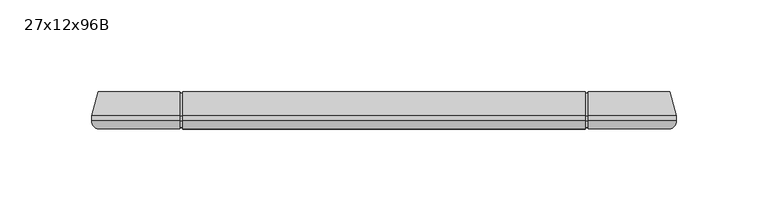
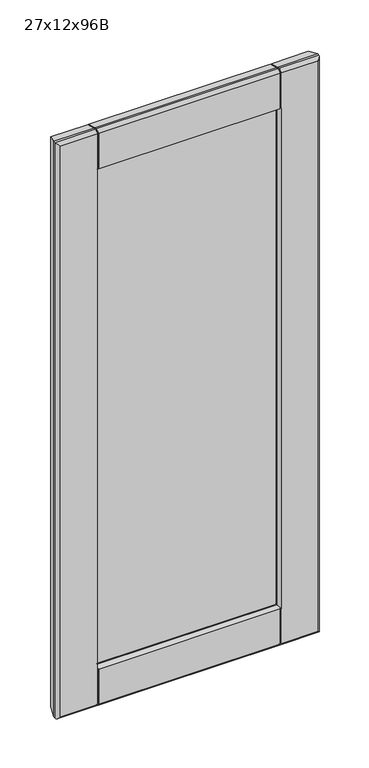
"""IFC4 building model written with IfcOpenShell, lengths in millimetres: furniture geometry, Cabinet-Tall-Merillat-Utility_Double-Marlin : 27x12x96B."""

from ifc_helpers import new_model, si_unit, frame, origin, place, context, project, spatial, polyline, circle_curve, ellipse_curve, outline, extrude, source, transform, mapped, element, save
from ifc_brep_helpers import plane_surface, cylinder_surface, advanced_brep


def furniture_27x12x96b_cd454a86(model_context):
    return source(origin(), model_context, "Body", "SolidModel", [
        advanced_brep(
        [(-326.6853408, -320.6496, 1676.4), (-323.5888483, -325.12, 1679.4964925), (-323.5888483, -325.12, 2409.9035075), (-326.6853408, -320.6496, 2413.0), (-326.6853408, -317.881, 2413.0), (-326.6853408, -317.881, 1676.4), (-323.1801408, -304.8, 2409.4948), (-323.1801408, -304.8, 1679.9052), (-278.4841781, -304.8, 1724.6011628), (-278.4841781, -304.8, 2364.7988372), (-278.1140464, -305.59375, 2364.4287055), (-276.0328873, -310.05681, 2362.3475465), (-276.0328873, -310.05681, 1727.0524535), (-278.1140464, -305.59375, 1724.9712945), (-277.4326568, -312.2969093, 2363.747316), (-277.4326568, -312.2969093, 1725.652684), (-291.7603408, -312.547, 2378.075), (-291.7603408, -312.547, 1711.325), (-291.7603408, -317.373, 2378.075), (-291.7603408, -317.373, 1711.325), (-277.4326568, -317.6230907, 2363.747316), (-277.4326568, -317.6230907, 1725.652684), (-276.0328873, -319.86319, 2362.3475465), (-276.0328873, -319.86319, 1727.0524535), (-278.1140464, -324.32625, 2364.4287055), (-278.4813106, -325.1138508, 2364.7959698), (-278.4841781, -325.12, 1724.6011628), (-278.1140464, -324.32625, 1724.9712945), (-278.4813106, -325.12, 2409.9035075), (-278.4813106, -320.6496, 2413.0), (-10.6943333, -325.12, 2409.9035075), (-7.5978408, -320.6496, 2413.0), (-55.7620595, -320.6496, 2413.0), (-55.7620595, -325.12, 2409.9035075), (-276.8938106, -320.6496, 2413.0), (-276.8938106, -325.12, 2409.9035075), (-57.3495595, -325.12, 2409.9035075), (-57.3495595, -320.6496, 2413.0), (-278.4813106, -317.881, 2413.0), (-7.5978408, -317.881, 2413.0), (-55.7620595, -317.881, 2413.0), (-276.8938106, -317.881, 2413.0), (-57.3495595, -317.881, 2413.0), (-278.4813106, -304.8, 2409.4948), (-11.1030408, -304.8, 2409.4948), (-55.7620595, -304.8, 2409.4948), (-276.8938106, -304.8, 2409.4948), (-57.3495595, -304.8, 2409.4948), (-58.2502943, -310.05681, 2362.3475465), (-276.8938106, -305.59375, 2364.4287055), (-276.8938106, -304.8, 2364.7988372), (-57.3495595, -304.8, 2364.7988372), (-57.3495595, -305.59375, 2364.4287055), (-56.1691353, -305.59375, 2364.4287055), (-56.8505249, -312.2969093, 2363.747316), (-42.5228408, -312.547, 2378.075), (-42.5228408, -317.373, 2378.075), (-56.8505249, -317.6230907, 2363.747316), (-58.2502943, -319.86319, 2362.3475465), (-56.1691353, -324.32625, 2364.4287055), (-57.3495595, -324.32625, 2364.4287055), (-57.3495595, -325.12, 2364.7988372), (-276.8938106, -325.12, 2364.7988372), (-276.8938106, -324.32625, 2364.4287055), (-10.6943333, -325.12, 1679.4964925), (-7.5978408, -320.6496, 1676.4), (-7.5978408, -317.881, 1676.4), (-11.1030408, -304.8, 1679.9052), (-55.7990036, -304.8, 2364.7988372), (-55.7990036, -304.8, 1724.6011628), (-56.1691353, -305.59375, 1724.9712945), (-58.2502943, -310.05681, 1727.0524535), (-56.8505249, -312.2969093, 1725.652684), (-42.5228408, -312.547, 1711.325), (-42.5228408, -317.373, 1711.325), (-56.8505249, -317.6230907, 1725.652684), (-58.2502943, -319.86319, 1727.0524535), (-56.1691353, -324.32625, 1724.9712945), (-55.7990036, -325.12, 1724.6011628), (-55.7990036, -325.12, 2364.7988372), (-55.7620595, -325.12, 1679.4964925), (-55.7620595, -320.6496, 1676.4), (-278.4813106, -320.6496, 1676.4), (-278.4813106, -325.12, 1679.4964925), (-57.3495595, -320.6496, 1676.4), (-57.3495595, -325.12, 1679.4964925), (-276.8938106, -325.12, 1679.4964925), (-276.8938106, -320.6496, 1676.4), (-55.7620595, -317.881, 1676.4), (-278.4813106, -317.881, 1676.4), (-57.3495595, -317.881, 1676.4), (-276.8938106, -317.881, 1676.4), (-55.7620595, -304.8, 1679.9052), (-278.4813106, -304.8, 1679.9052), (-57.3495595, -304.8, 1679.9052), (-276.8938106, -304.8, 1679.9052), (-57.3495595, -304.8, 1724.6011628), (-276.8938106, -304.8, 1724.6011628), (-57.3495595, -305.59375, 1724.9712945), (-276.8938106, -305.59375, 1724.9712945), (-276.8938106, -324.32625, 1724.9712945), (-276.8938106, -325.12, 1724.6011628), (-57.3495595, -325.12, 1724.6011628), (-57.3495595, -324.32625, 1724.9712945), (-57.3495595, -305.59375, 1680.5142588), (-57.3495595, -317.9855037, 1677.19375), (-57.3495595, -320.6496, 1677.19375), (-57.3495595, -324.32625, 1679.6473948), (-55.7620595, -324.32625, 1724.9712945), (-55.7620595, -324.32625, 1679.6473948), (-55.7620595, -320.6496, 1677.19375), (-55.7620595, -317.9855037, 1677.19375), (-55.7620595, -305.59375, 1680.5142588), (-55.7620595, -305.59375, 1724.9712945), (-278.4813106, -305.59375, 1724.9712945), (-278.4813106, -305.59375, 1680.5142588), (-278.4813106, -317.9855037, 1677.19375), (-278.4813106, -320.6496, 1677.19375), (-278.4813106, -324.32625, 1679.6473948), (-278.4813106, -324.32625, 1724.9712945), (-276.8938106, -324.32625, 1679.6473948), (-276.8938106, -320.6496, 1677.19375), (-276.8938106, -317.9855037, 1677.19375), (-276.8938106, -305.59375, 1680.5142588), (-278.4813106, -324.32625, 2364.4287055), (-278.4813106, -324.32625, 2409.7526052), (-278.4813106, -320.6496, 2412.20625), (-278.4813106, -317.9855037, 2412.20625), (-278.4813106, -305.59375, 2408.8857412), (-278.4813106, -305.59375, 2364.4287055), (-276.8938106, -305.59375, 2408.8857412), (-276.8938106, -317.9855037, 2412.20625), (-276.8938106, -320.6496, 2412.20625), (-276.8938106, -324.32625, 2409.7526052), (-57.3495595, -324.32625, 2409.7526052), (-57.3495595, -320.6496, 2412.20625), (-57.3495595, -317.9855037, 2412.20625), (-57.3495595, -305.59375, 2408.8857412), (-55.7620595, -324.32625, 2364.4287055), (-55.7620595, -305.59375, 2364.4287055), (-55.7620595, -305.59375, 2408.8857412), (-55.7620595, -317.9855037, 2412.20625), (-55.7620595, -320.6496, 2412.20625), (-55.7620595, -324.32625, 2409.7526052)],
        [
            (0, 1, ellipse_curve(frame((-321.9101408, -320.6496, 1681.1752), z_axis=(-0.7071067811865505, 0.0, 0.7071067811865446), x_axis=(-0.7071067811865445, 0.0, -0.7071067811865505)), 6.7531526, 4.7752)),
            (1, 2),
            (2, 3, ellipse_curve(frame((-321.9101408, -320.6496, 2408.2248), z_axis=(-0.7071067811865446, 0.0, -0.7071067811865505), x_axis=(0.7071067811865505, 0.0, -0.7071067811865445)), 6.7531526, 4.7752)),
            (3, 0),
            (3, 4),
            (4, 5),
            (5, 0),
            (4, 6),
            (6, 7),
            (7, 5),
            (8, 9),
            (9, 10),
            (10, 11),
            (11, 12),
            (12, 13),
            (13, 8),
            (11, 14, ellipse_curve(frame((-277.4601408, -310.7223492, 2363.7748), z_axis=(-0.7071067811865446, 0.0, -0.7071067811865505), x_axis=(0.7071067811865505, 0.0, -0.7071067811865445)), 2.2271035, 1.5748)),
            (14, 15),
            (15, 12, ellipse_curve(frame((-277.4601408, -310.7223492, 1725.6252), z_axis=(-0.7071067811865505, 0.0, 0.7071067811865446), x_axis=(-0.7071067811865445, 0.0, -0.7071067811865505)), 2.2271035, 1.5748)),
            (14, 16),
            (16, 17),
            (17, 15),
            (16, 18),
            (18, 19),
            (19, 17),
            (18, 20),
            (20, 21),
            (21, 19),
            (20, 22, ellipse_curve(frame((-277.4601408, -319.1976508, 2363.7748), z_axis=(-0.7071067811865446, 0.0, -0.7071067811865505), x_axis=(0.7071067811865505, 0.0, -0.7071067811865445)), 2.2271035, 1.5748)),
            (22, 23),
            (23, 21, ellipse_curve(frame((-277.4601408, -319.1976508, 1725.6252), z_axis=(-0.7071067811865505, 0.0, 0.7071067811865446), x_axis=(-0.7071067811865445, 0.0, -0.7071067811865505)), 2.2271035, 1.5748)),
            (22, 24),
            (24, 25),
            (25, 26),
            (26, 27),
            (27, 23),
            (2, 28),
            (28, 29, circle_curve(frame((-278.4813106, -320.6496, 2408.2248), z_axis=(-1.0, 0.0, 0.0), x_axis=(0.0, 1.0, 0.0)), 4.7752)),
            (29, 3),
            (30, 31, ellipse_curve(frame((-12.3730408, -320.6496, 2408.2248), z_axis=(-0.7071067811865505, 0.0, 0.7071067811865446), x_axis=(-0.7071067811865445, 0.0, -0.7071067811865505)), 6.7531526, 4.7752)),
            (31, 32),
            (32, 33, circle_curve(frame((-55.7620595, -320.6496, 2408.2248), z_axis=(1.0, 0.0, 0.0), x_axis=(0.0, 1.0, 0.0)), 4.7752)),
            (33, 30),
            (34, 35, circle_curve(frame((-276.8938106, -320.6496, 2408.2248), z_axis=(1.0, 0.0, 0.0), x_axis=(0.0, 1.0, 0.0)), 4.7752)),
            (35, 36),
            (36, 37, circle_curve(frame((-57.3495595, -320.6496, 2408.2248), z_axis=(-1.0, 0.0, 0.0), x_axis=(0.0, 1.0, 0.0)), 4.7752)),
            (37, 34),
            (29, 38),
            (38, 4),
            (31, 39),
            (39, 40),
            (40, 32),
            (41, 34),
            (37, 42),
            (42, 41),
            (38, 43),
            (43, 6),
            (39, 44),
            (44, 45),
            (45, 40),
            (46, 41),
            (42, 47),
            (47, 46),
            (48, 11),
            (10, 49),
            (49, 50),
            (50, 51),
            (51, 52),
            (52, 53),
            (53, 48),
            (48, 54, ellipse_curve(frame((-56.8230408, -310.7223492, 2363.7748), z_axis=(-0.7071067811865505, 0.0, 0.7071067811865446), x_axis=(-0.7071067811865445, 0.0, -0.7071067811865505)), 2.2271035, 1.5748)),
            (54, 14),
            (54, 55),
            (55, 16),
            (55, 56),
            (56, 18),
            (56, 57),
            (57, 20),
            (57, 58, ellipse_curve(frame((-56.8230408, -319.1976508, 2363.7748), z_axis=(-0.7071067811865505, 0.0, 0.7071067811865446), x_axis=(-0.7071067811865445, 0.0, -0.7071067811865505)), 2.2271035, 1.5748)),
            (58, 22),
            (58, 59),
            (59, 60),
            (60, 61),
            (61, 62),
            (62, 63),
            (63, 24),
            (30, 64),
            (64, 65, ellipse_curve(frame((-12.3730408, -320.6496, 1681.1752), z_axis=(0.7071067811865446, 0.0, 0.7071067811865505), x_axis=(-0.7071067811865505, 0.0, 0.7071067811865445)), 6.7531526, 4.7752)),
            (65, 31),
            (65, 66),
            (66, 39),
            (66, 67),
            (67, 44),
            (68, 69),
            (69, 70),
            (70, 71),
            (71, 48),
            (53, 68),
            (71, 72, ellipse_curve(frame((-56.8230408, -310.7223492, 1725.6252), z_axis=(0.7071067811865446, 0.0, 0.7071067811865505), x_axis=(-0.7071067811865505, 0.0, 0.7071067811865445)), 2.2271035, 1.5748)),
            (72, 54),
            (72, 73),
            (73, 55),
            (73, 74),
            (74, 56),
            (74, 75),
            (75, 57),
            (75, 76, ellipse_curve(frame((-56.8230408, -319.1976508, 1725.6252), z_axis=(0.7071067811865446, 0.0, 0.7071067811865505), x_axis=(-0.7071067811865505, 0.0, 0.7071067811865445)), 2.2271035, 1.5748)),
            (76, 58),
            (76, 77),
            (77, 78),
            (78, 79),
            (79, 59),
            (64, 80),
            (80, 81, circle_curve(frame((-55.7620595, -320.6496, 1681.1752), z_axis=(1.0, 0.0, 0.0), x_axis=(0.0, 1.0, 0.0)), 4.7752)),
            (81, 65),
            (0, 82),
            (82, 83, circle_curve(frame((-278.4813106, -320.6496, 1681.1752), z_axis=(-1.0, 0.0, 0.0), x_axis=(0.0, 1.0, 0.0)), 4.7752)),
            (83, 1),
            (84, 85, circle_curve(frame((-57.3495595, -320.6496, 1681.1752), z_axis=(-1.0, 0.0, 0.0), x_axis=(0.0, 1.0, 0.0)), 4.7752)),
            (85, 86),
            (86, 87, circle_curve(frame((-276.8938106, -320.6496, 1681.1752), z_axis=(1.0, 0.0, 0.0), x_axis=(0.0, 1.0, 0.0)), 4.7752)),
            (87, 84),
            (81, 88),
            (88, 66),
            (5, 89),
            (89, 82),
            (90, 84),
            (87, 91),
            (91, 90),
            (88, 92),
            (92, 67),
            (7, 93),
            (93, 89),
            (94, 90),
            (91, 95),
            (95, 94),
            (43, 9),
            (8, 93),
            (92, 69),
            (68, 45),
            (96, 94),
            (95, 97),
            (97, 96),
            (50, 46),
            (47, 51),
            (12, 71),
            (70, 98),
            (98, 96),
            (97, 99),
            (99, 13),
            (15, 72),
            (17, 73),
            (19, 74),
            (21, 75),
            (23, 76),
            (27, 100),
            (100, 101),
            (101, 102),
            (102, 103),
            (103, 77),
            (83, 26),
            (25, 28),
            (33, 79),
            (78, 80),
            (85, 102),
            (101, 86),
            (35, 62),
            (61, 36),
            (98, 104),
            (104, 105),
            (105, 106),
            (106, 107, circle_curve(frame((-57.3495595, -320.6496, 1681.1752), z_axis=(-1.0, 0.0, 0.0), x_axis=(0.0, 0.0, -1.0)), 3.98145)),
            (107, 103),
            (78, 108),
            (108, 109),
            (109, 110, circle_curve(frame((-55.7620595, -320.6496, 1681.1752), z_axis=(1.0, 0.0, 0.0), x_axis=(0.0, 0.0, -1.0)), 3.98145)),
            (110, 111),
            (111, 112),
            (112, 113),
            (113, 69),
            (77, 108),
            (107, 109),
            (106, 110),
            (105, 111),
            (104, 112),
            (70, 113),
            (8, 114),
            (114, 115),
            (115, 116),
            (116, 117),
            (117, 118, circle_curve(frame((-278.4813106, -320.6496, 1681.1752), z_axis=(-1.0, 0.0, 0.0), x_axis=(0.0, 0.0, -1.0)), 3.98145)),
            (118, 119),
            (119, 26),
            (100, 120),
            (120, 121, circle_curve(frame((-276.8938106, -320.6496, 1681.1752), z_axis=(1.0, 0.0, 0.0), x_axis=(0.0, 0.0, -1.0)), 3.98145)),
            (121, 122),
            (122, 123),
            (123, 99),
            (119, 27),
            (118, 120),
            (117, 121),
            (116, 122),
            (115, 123),
            (114, 13),
            (25, 124),
            (124, 125),
            (125, 126, circle_curve(frame((-278.4813106, -320.6496, 2408.2248), z_axis=(-1.0, 0.0, 0.0), x_axis=(0.0, 0.0, -1.0)), 3.98145)),
            (126, 127),
            (127, 128),
            (128, 129),
            (129, 9),
            (49, 130),
            (130, 131),
            (131, 132),
            (132, 133, circle_curve(frame((-276.8938106, -320.6496, 2408.2248), z_axis=(1.0, 0.0, 0.0), x_axis=(0.0, 0.0, -1.0)), 3.98145)),
            (133, 63),
            (129, 10),
            (128, 130),
            (127, 131),
            (126, 132),
            (125, 133),
            (124, 24),
            (60, 134),
            (134, 135, circle_curve(frame((-57.3495595, -320.6496, 2408.2248), z_axis=(-1.0, 0.0, 0.0), x_axis=(0.0, 0.0, -1.0)), 3.98145)),
            (135, 136),
            (136, 137),
            (137, 52),
            (138, 79),
            (68, 139),
            (139, 140),
            (140, 141),
            (141, 142),
            (142, 143, circle_curve(frame((-55.7620595, -320.6496, 2408.2248), z_axis=(1.0, 0.0, 0.0), x_axis=(0.0, 0.0, -1.0)), 3.98145)),
            (143, 138),
            (138, 59),
            (53, 139),
            (137, 140),
            (136, 141),
            (135, 142),
            (134, 143),
        ],
        [
            cylinder_surface(frame((-321.9101408, -320.6496, 1676.4), z_axis=(0.0, 0.0, -1.0), x_axis=(0.0, 1.0, 0.0)), 4.7752),
            plane_surface(frame((-326.6853408, -320.6496, 1676.4), z_axis=(-1.0, 0.0, 0.0), x_axis=(0.0, 0.0, 1.0))),
            plane_surface(frame((-326.6853408, -317.881, 1676.4), z_axis=(-0.9659229350723619, 0.25882983502910506, 0.0), x_axis=(0.0, 0.0, 1.0))),
            plane_surface(frame((-278.4841781, -304.8, 1724.6011628), z_axis=(0.9063077870366099, 0.4226182617407856, 0.0), x_axis=(0.0, 0.0, 1.0))),
            cylinder_surface(frame((-277.4601408, -310.7223492, 1676.4), z_axis=(0.0, 0.0, -1.0000000000000002), x_axis=(0.01745240643729364, -0.9998476951563912, 0.0)), 1.5748),
            plane_surface(frame((-277.4326568, -312.2969093, 1725.652684), z_axis=(0.017452406437322144, -0.9998476951563906, 0.0), x_axis=(0.0, 0.0, 1.0))),
            plane_surface(frame((-291.7603408, -312.547, 1711.325), z_axis=(1.0, 0.0, 0.0), x_axis=(0.0, 0.0, 1.0))),
            plane_surface(frame((-291.7603408, -317.373, 1711.325), z_axis=(0.01745240643727848, 0.9998476951563914, 0.0), x_axis=(0.0, 0.0, 1.0))),
            cylinder_surface(frame((-277.4601408, -319.1976508, 1676.4), z_axis=(0.0, 0.0, -1.0000000000000002), x_axis=(0.9063077870367326, -0.42261826174052236, 0.0)), 1.5748),
            plane_surface(frame((-276.0328873, -319.86319, 1727.0524535), z_axis=(0.9063077870366333, -0.4226182617407352, 0.0), x_axis=(0.0, 0.0, 1.0))),
            cylinder_surface(frame((-326.6853408, -320.6496, 2408.2248), z_axis=(-1.0, 0.0, 0.0), x_axis=(0.0, 1.0, 0.0)), 4.7752),
            plane_surface(frame((-326.6853408, -320.6496, 2413.0), z_axis=(0.0, 0.0, 1.0), x_axis=(1.0, 0.0, 0.0))),
            plane_surface(frame((-326.6853408, -317.881, 2413.0), z_axis=(0.0, 0.25882983502910506, 0.9659229350723619), x_axis=(1.0, 0.0, 0.0))),
            plane_surface(frame((-278.4841781, -304.8, 2364.7988372), z_axis=(0.0, 0.4226182617407856, -0.9063077870366099), x_axis=(1.0, 0.0, 0.0))),
            cylinder_surface(frame((-326.6853408, -310.7223492, 2363.7748), z_axis=(-1.0000000000000002, 0.0, 0.0), x_axis=(0.0, -0.9998476951563912, -0.01745240643729364)), 1.5748),
            plane_surface(frame((-277.4326568, -312.2969093, 2363.747316), z_axis=(0.0, -0.9998476951563906, -0.017452406437322144), x_axis=(1.0, 0.0, 0.0))),
            plane_surface(frame((-291.7603408, -312.547, 2378.075), z_axis=(0.0, 0.0, -1.0), x_axis=(1.0, 0.0, 0.0))),
            plane_surface(frame((-291.7603408, -317.373, 2378.075), z_axis=(0.0, 0.9998476951563914, -0.01745240643727848), x_axis=(1.0, 0.0, 0.0))),
            cylinder_surface(frame((-326.6853408, -319.1976508, 2363.7748), z_axis=(-1.0000000000000002, 0.0, 0.0), x_axis=(0.0, -0.42261826174052236, -0.9063077870367326)), 1.5748),
            plane_surface(frame((-276.0328873, -319.86319, 2362.3475465), z_axis=(0.0, -0.4226182617407352, -0.9063077870366333), x_axis=(1.0, 0.0, 0.0))),
            cylinder_surface(frame((-12.3730408, -320.6496, 2413.0), z_axis=(0.0, 0.0, 1.0), x_axis=(0.0, 1.0, 0.0)), 4.7752),
            plane_surface(frame((-7.5978408, -320.6496, 2413.0), z_axis=(1.0, 0.0, 0.0), x_axis=(0.0, 0.0, -1.0))),
            plane_surface(frame((-7.5978408, -317.881, 2413.0), z_axis=(0.9659229350723619, 0.25882983502910506, 0.0), x_axis=(0.0, 0.0, -1.0))),
            plane_surface(frame((-55.7990036, -304.8, 2364.7988372), z_axis=(-0.9063077870366099, 0.4226182617407856, 0.0), x_axis=(0.0, 0.0, -1.0))),
            cylinder_surface(frame((-56.8230408, -310.7223492, 2413.0), z_axis=(0.0, 0.0, 1.0000000000000002), x_axis=(-0.01745240643729364, -0.9998476951563912, 0.0)), 1.5748),
            plane_surface(frame((-56.8505249, -312.2969093, 2363.747316), z_axis=(-0.017452406437322144, -0.9998476951563906, 0.0), x_axis=(0.0, 0.0, -1.0))),
            plane_surface(frame((-42.5228408, -312.547, 2378.075), z_axis=(-1.0, 0.0, 0.0), x_axis=(0.0, 0.0, -1.0))),
            plane_surface(frame((-42.5228408, -317.373, 2378.075), z_axis=(-0.01745240643727848, 0.9998476951563914, 0.0), x_axis=(0.0, 0.0, -1.0))),
            cylinder_surface(frame((-56.8230408, -319.1976508, 2413.0), z_axis=(0.0, 0.0, 1.0000000000000002), x_axis=(-0.9063077870367326, -0.42261826174052236, 0.0)), 1.5748),
            plane_surface(frame((-58.2502943, -319.86319, 2362.3475465), z_axis=(-0.9063077870366333, -0.4226182617407352, 0.0), x_axis=(0.0, 0.0, -1.0))),
            cylinder_surface(frame((-7.5978408, -320.6496, 1681.1752), z_axis=(1.0, 0.0, 0.0), x_axis=(0.0, 1.0, 0.0)), 4.7752),
            plane_surface(frame((-7.5978408, -320.6496, 1676.4), z_axis=(0.0, 0.0, -1.0), x_axis=(-1.0, 0.0, 0.0))),
            plane_surface(frame((-7.5978408, -317.881, 1676.4), z_axis=(0.0, 0.25882983502910506, -0.9659229350723619), x_axis=(-1.0, 0.0, 0.0))),
            plane_surface(frame((-11.1030408, -304.8, 1679.9052), z_axis=(0.0, 1.0, 0.0), x_axis=(-1.0, 0.0, 0.0))),
            plane_surface(frame((-55.7990036, -304.8, 1724.6011628), z_axis=(0.0, 0.4226182617407856, 0.9063077870366099), x_axis=(-1.0, 0.0, 0.0))),
            cylinder_surface(frame((-7.5978408, -310.7223492, 1725.6252), z_axis=(1.0000000000000002, 0.0, 0.0), x_axis=(0.0, -0.9998476951563912, 0.01745240643729364)), 1.5748),
            plane_surface(frame((-56.8505249, -312.2969093, 1725.652684), z_axis=(0.0, -0.9998476951563906, 0.017452406437322144), x_axis=(-1.0, 0.0, 0.0))),
            plane_surface(frame((-42.5228408, -312.547, 1711.325), z_axis=(0.0, 0.0, 1.0), x_axis=(-1.0, 0.0, 0.0))),
            plane_surface(frame((-42.5228408, -317.373, 1711.325), z_axis=(0.0, 0.9998476951563914, 0.01745240643727848), x_axis=(-1.0, 0.0, 0.0))),
            cylinder_surface(frame((-7.5978408, -319.1976508, 1725.6252), z_axis=(1.0000000000000002, 0.0, 0.0), x_axis=(0.0, -0.42261826174052236, 0.9063077870367326)), 1.5748),
            plane_surface(frame((-58.2502943, -319.86319, 1727.0524535), z_axis=(0.0, -0.4226182617407352, 0.9063077870366333), x_axis=(-1.0, 0.0, 0.0))),
            plane_surface(frame((-55.7990036, -325.12, 1724.6011628), z_axis=(0.0, -1.0, 0.0), x_axis=(-1.0, 0.0, 0.0))),
            plane_surface(frame((-57.3495595, -325.12, 1724.6011628), z_axis=(1.0000000000000002, 0.0, 0.0), x_axis=(0.0, 0.9063077870366255, 0.4226182617407521))),
            plane_surface(frame((-55.7620595, -325.12, 1724.6011628), z_axis=(-1.0000000000000002, 0.0, 0.0), x_axis=(0.0, -0.9063077870366255, -0.4226182617407521))),
            plane_surface(frame((-57.3495595, -325.12, 1724.6011628), z_axis=(0.0, 0.4226182617407521, -0.9063077870366255), x_axis=(1.0, 0.0, 0.0))),
            plane_surface(frame((-57.3495595, -324.32625, 1724.9712945), z_axis=(0.0, -1.0, 0.0), x_axis=(1.0, 0.0, 0.0))),
            cylinder_surface(frame((-55.7620595, -320.6496, 1681.1752), z_axis=(1.0, 0.0, 0.0), x_axis=(0.0, 0.0, -1.0)), 3.98145),
            plane_surface(frame((-57.3495595, -320.6496, 1677.19375), z_axis=(0.0, 0.0, -1.0), x_axis=(1.0, 0.0, 0.0))),
            plane_surface(frame((-57.3495595, -317.9855037, 1677.19375), z_axis=(0.0, 0.25882983502916707, -0.9659229350723454), x_axis=(1.0, 0.0, 0.0))),
            plane_surface(frame((-57.3495595, -305.59375, 1680.5142588), z_axis=(0.0, 1.0, 0.0), x_axis=(1.0, 0.0, 0.0))),
            plane_surface(frame((-57.3495595, -305.59375, 1724.9712945), z_axis=(0.0, -0.42261826174074746, -0.9063077870366276), x_axis=(1.0, 0.0, 0.0))),
            plane_surface(frame((-278.4813106, -325.12, 1724.6011628), z_axis=(1.0, 0.0, 0.0), x_axis=(0.0, 0.9063077870366341, 0.4226182617407336))),
            plane_surface(frame((-276.8938106, -325.12, 1724.6011628), z_axis=(-1.0, 0.0, 0.0), x_axis=(0.0, -0.9063077870366341, -0.4226182617407336))),
            plane_surface(frame((-278.4813106, -325.12, 1724.6011628), z_axis=(0.0, 0.4226182617407336, -0.9063077870366341), x_axis=(1.0, 0.0, 0.0))),
            plane_surface(frame((-278.4813106, -324.32625, 1724.9712945), z_axis=(0.0, -1.0, 0.0), x_axis=(1.0, 0.0, 0.0))),
            cylinder_surface(frame((-276.8938106, -320.6496, 1681.1752), z_axis=(1.0, 0.0, 0.0), x_axis=(0.0, 0.0, -1.0)), 3.98145),
            plane_surface(frame((-278.4813106, -320.6496, 1677.19375), z_axis=(0.0, 0.0, -1.0), x_axis=(1.0, 0.0, 0.0))),
            plane_surface(frame((-278.4813106, -317.9855037, 1677.19375), z_axis=(0.0, 0.25882983502916396, -0.9659229350723462), x_axis=(1.0, 0.0, 0.0))),
            plane_surface(frame((-278.4813106, -305.59375, 1680.5142588), z_axis=(0.0, 1.0, 0.0), x_axis=(1.0, 0.0, 0.0))),
            plane_surface(frame((-278.4813106, -305.59375, 1724.9712945), z_axis=(0.0, -0.4226182617407683, -0.9063077870366179), x_axis=(1.0, 0.0, 0.0))),
            plane_surface(frame((-278.4813106, -320.6496, 2403.4496), z_axis=(1.0, 0.0, 0.0), x_axis=(0.0, -1.0, 0.0))),
            plane_surface(frame((-276.8938106, -320.6496, 2403.4496), z_axis=(-1.0, 0.0, 0.0), x_axis=(0.0, 1.0, 0.0))),
            plane_surface(frame((-278.4813106, -304.8, 2364.7988372), z_axis=(0.0, -0.42261826174076006, 0.9063077870366217), x_axis=(1.0, 0.0, 0.0))),
            plane_surface(frame((-278.4813106, -305.59375, 2364.4287055), z_axis=(0.0, 1.0, 0.0), x_axis=(1.0, 0.0, 0.0))),
            plane_surface(frame((-278.4813106, -305.59375, 2408.8857412), z_axis=(0.0, 0.2588298350294376, 0.9659229350722728), x_axis=(1.0, 0.0, 0.0))),
            plane_surface(frame((-278.4813106, -317.9855037, 2412.20625), z_axis=(0.0, 0.0, 1.0), x_axis=(1.0, 0.0, 0.0))),
            cylinder_surface(frame((-276.8938106, -320.6496, 2408.2248), z_axis=(1.0, 0.0, 0.0), x_axis=(0.0, 0.0, -1.0)), 3.98145),
            plane_surface(frame((-278.4813106, -324.32625, 2409.7526052), z_axis=(0.0, -1.0, 0.0), x_axis=(1.0, 0.0, 0.0))),
            plane_surface(frame((-278.4813106, -324.32625, 2364.4287055), z_axis=(0.0, 0.42261826174073647, 0.9063077870366327), x_axis=(1.0, 0.0, 0.0))),
            plane_surface(frame((-57.3495595, -324.32625, 2364.4287055), z_axis=(1.0, 0.0, 0.0), x_axis=(0.0, -0.9063077870366145, 0.42261826174077555))),
            plane_surface(frame((-55.7620595, -324.32625, 2364.4287055), z_axis=(-1.0, 0.0, 0.0), x_axis=(0.0, 0.9063077870366145, -0.42261826174077555))),
            plane_surface(frame((-57.3495595, -324.32625, 2364.4287055), z_axis=(0.0, 0.42261826174077555, 0.9063077870366145), x_axis=(1.0, 0.0, 0.0))),
            plane_surface(frame((-57.3495595, -304.8, 2364.7988372), z_axis=(0.0, -0.4226182617407416, 0.9063077870366304), x_axis=(1.0, 0.0, 0.0))),
            plane_surface(frame((-57.3495595, -305.59375, 2364.4287055), z_axis=(0.0, 1.0, 0.0), x_axis=(1.0, 0.0, 0.0))),
            plane_surface(frame((-57.3495595, -305.59375, 2408.8857412), z_axis=(0.0, 0.2588298350294381, 0.9659229350722727), x_axis=(1.0, 0.0, 0.0))),
            plane_surface(frame((-57.3495595, -317.9855037, 2412.20625), z_axis=(0.0, 0.0, 1.0), x_axis=(1.0, 0.0, 0.0))),
            cylinder_surface(frame((-55.7620595, -320.6496, 2408.2248), z_axis=(1.0, 0.0, 0.0), x_axis=(0.0, 0.0, -1.0)), 3.98145),
            plane_surface(frame((-57.3495595, -324.32625, 2409.7526052), z_axis=(0.0, -1.0, 0.0), x_axis=(1.0, 0.0, 0.0))),
        ],
        [
            (0, [[1, 2, 3, 4]]),
            (1, [[-4, 5, 6, 7]]),
            (2, [[-6, 8, 9, 10]]),
            (3, [[11, 12, 13, 14, 15, 16]]),
            (4, [[-14, 17, 18, 19]]),
            (5, [[-18, 20, 21, 22]]),
            (6, [[-21, 23, 24, 25]]),
            (7, [[-24, 26, 27, 28]]),
            (8, [[-27, 29, 30, 31]]),
            (9, [[-30, 32, 33, 34, 35, 36]]),
            (10, [[-3, 37, 38, 39]]),
            (10, [[40, 41, 42, 43]]),
            (10, [[44, 45, 46, 47]]),
            (11, [[-5, -39, 48, 49]]),
            (11, [[50, 51, 52, -41]]),
            (11, [[53, -47, 54, 55]]),
            (12, [[-8, -49, 56, 57]]),
            (12, [[58, 59, 60, -51]]),
            (12, [[61, -55, 62, 63]]),
            (13, [[64, -13, 65, 66, 67, 68, 69, 70]]),
            (14, [[-17, -64, 71, 72]]),
            (15, [[-20, -72, 73, 74]]),
            (16, [[-23, -74, 75, 76]]),
            (17, [[-26, -76, 77, 78]]),
            (18, [[-29, -78, 79, 80]]),
            (19, [[-80, 81, 82, 83, 84, 85, 86, -32]]),
            (20, [[-40, 87, 88, 89]]),
            (21, [[-50, -89, 90, 91]]),
            (22, [[-58, -91, 92, 93]]),
            (23, [[94, 95, 96, 97, -70, 98]]),
            (24, [[-71, -97, 99, 100]]),
            (25, [[-73, -100, 101, 102]]),
            (26, [[-75, -102, 103, 104]]),
            (27, [[-77, -104, 105, 106]]),
            (28, [[-79, -106, 107, 108]]),
            (29, [[-108, 109, 110, 111, 112, -81]]),
            (30, [[-88, 113, 114, 115]]),
            (30, [[-1, 116, 117, 118]]),
            (30, [[119, 120, 121, 122]]),
            (31, [[-90, -115, 123, 124]]),
            (31, [[-7, 125, 126, -116]]),
            (31, [[127, -122, 128, 129]]),
            (32, [[-92, -124, 130, 131]]),
            (32, [[-10, 132, 133, -125]]),
            (32, [[134, -129, 135, 136]]),
            (33, [[-9, -57, 137, -11, 138, -132]]),
            (33, [[-93, -131, 139, -94, 140, -59]]),
            (33, [[141, -136, 142, 143]]),
            (33, [[144, -63, 145, -67]]),
            (34, [[146, -96, 147, 148, -143, 149, 150, -15]]),
            (35, [[-19, 151, -99, -146]]),
            (36, [[-22, 152, -101, -151]]),
            (37, [[-25, 153, -103, -152]]),
            (38, [[-28, 154, -105, -153]]),
            (39, [[-31, 155, -107, -154]]),
            (40, [[-155, -36, 156, 157, 158, 159, 160, -109]]),
            (41, [[-2, -118, 161, -34, 162, -37]]),
            (41, [[-87, -43, 163, -111, 164, -113]]),
            (41, [[165, -158, 166, -120]]),
            (41, [[167, -84, 168, -45]]),
            (42, [[169, 170, 171, 172, 173, -159, -165, -119, -127, -134, -141, -148]]),
            (43, [[174, 175, 176, 177, 178, 179, 180, -139, -130, -123, -114, -164]]),
            (44, [[-174, -110, 181]]),
            (45, [[-173, 182, -175, -181, -160]]),
            (46, [[-172, 183, -176, -182]]),
            (47, [[-171, 184, -177, -183]]),
            (48, [[-170, 185, -178, -184]]),
            (49, [[-169, -147, 186, -179, -185]]),
            (50, [[-180, -186, -95]]),
            (51, [[187, 188, 189, 190, 191, 192, 193, -161, -117, -126, -133, -138]]),
            (52, [[194, 195, 196, 197, 198, -149, -142, -135, -128, -121, -166, -157]]),
            (53, [[-193, 199, -35]]),
            (54, [[-192, 200, -194, -156, -199]]),
            (55, [[-191, 201, -195, -200]]),
            (56, [[-190, 202, -196, -201]]),
            (57, [[-189, 203, -197, -202]]),
            (58, [[-188, 204, -150, -198, -203]]),
            (59, [[-187, -16, -204]]),
            (60, [[205, 206, 207, 208, 209, 210, 211, -137, -56, -48, -38, -162]]),
            (61, [[212, 213, 214, 215, 216, -85, -167, -44, -53, -61, -144, -66]]),
            (62, [[-211, 217, -12]]),
            (63, [[-210, 218, -212, -65, -217]]),
            (64, [[-209, 219, -213, -218]]),
            (65, [[-208, 220, -214, -219]]),
            (66, [[-207, 221, -215, -220]]),
            (67, [[-206, 222, -86, -216, -221]]),
            (68, [[-205, -33, -222]]),
            (69, [[223, 224, 225, 226, 227, -68, -145, -62, -54, -46, -168, -83]]),
            (70, [[228, -163, -42, -52, -60, -140, 229, 230, 231, 232, 233, 234]]),
            (71, [[-228, 235, -112]]),
            (72, [[-229, -98, 236]]),
            (73, [[-227, 237, -230, -236, -69]]),
            (74, [[-226, 238, -231, -237]]),
            (75, [[-225, 239, -232, -238]]),
            (76, [[-224, 240, -233, -239]]),
            (77, [[-223, -82, -235, -234, -240]]),
        ],
    ),
        extrude(outline(polyline([(-42.5228408, -317.373), (-291.7603408, -317.373), (-291.7603408, -312.547), (-42.5228408, -312.547), (-42.5228408, -317.373)])), frame((0.0, 0.0, 1711.325), z_axis=(0.0, 0.0, 1.0), x_axis=(1.0, 0.0, 0.0)), (0.0, 0.0, 1.0), 666.75),
    ])


if __name__ == "__main__":
    model = new_model("IFC4")
    model_context = context("Model", 3, world=origin())
    ifc_project = project(units=[si_unit("LENGTHUNIT", "METRE", prefix="MILLI")], contexts=[model_context])
    site = spatial("IfcSite", under=ifc_project)
    building = spatial("IfcBuilding", under=site)
    placement = place(None, origin())
    furniture_27x12x96b_shape = furniture_27x12x96b_cd454a86(model_context)
    element("IfcFurniture", 1, ObjectType="Cabinet-Tall-Merillat-Utility_Double-Marlin : 27x12x96B", at=placement, inside=building, context=model_context, shape_type="MappedRepresentation", body=[
        mapped(furniture_27x12x96b_shape, transform((0.0, 0.0, 0.0), x_axis=(1.0, 0.0, 0.0), y_axis=(0.0, 1.0, 0.0), z_axis=(0.0, 0.0, 1.0))),
    ])
    save(model, "model.ifc")

# Revit data of these elements
# Type "Cabinet-Tall-Merillat-Utility_Double-Marlin : 27x12x96B"
#   URL = "http://www.merillat.com/"
#   Toe Kick Note = "Toe Kick Covering is not included. To be purchased Separately. \r\n\r\n Toe Kick Covering is not included. To be purchased Separately."
#   Product Page URL = "http://www.merillat.com/our-products/rooms/kitchen/"
#   Product Line = "Express"
#   Product Group = "Tall Cabinet"
#   Product Documentation Link = "http://merillatbusiness.com/wp-content/uploads/2014/07/Merillat_Classic_Catalog.pdf"
#   Model = "U3096B"
#   Manufacturer = "Merillat"
#   Finish = "Wood"
#   Description = "Tall Utility Cabinet Double"
#   Construction Type = "Tall Cabinet"
#   Cabinet Construction Note = ""
#   Assembly Code = "C1030410"
#   Spacing = 0' - 1"
#   Door Spacing = 0' - 0 1/8"
#   Cabinet Upper Door Height = 2' - 5"
#   Cabinet Door Width = 1' - 0 9/16"
#   Cabinet Door Height = 4' - 11 1/2"
#   Depth = 1' - 0"
#   Height = 8' - 0"
#   Toe Depth = 0' - 2 25/32"
#   Toe Height = 0' - 4 1/2"
#   Width = 2' - 3"
#   COBie.Type = no
#   Partial Overlay Butt = yes
#   Partial Overlay = no
#   Full Overlay Butt = no
#   Full Overlay = no
#   Elevation Swing Line = yes
#   Toe Kick Material = Wood - Merillat - Raw Particle Board
#   Door Drawer Material = Wood - Merillat - Pecan(1)
#   Cabinet Material = Wood - Merillat - Pecan(1)
#   Cabinet Door Style = element 776454
# Element 1 (IfcFurniture, "Cabinet-Tall-Merillat-Utility_Double-Marlin : 27x12x96B")
#   Materials on its faces: "Wood - Merillat - Pecan(1)", "Wood - Merillat - Raw Particle Board"
# Materials
#   "Wood - Merillat - Raw Particle Board": class "Plastic", colour RGB 80 80 80, transparency 0, Description = "Plastic Laminate - Navy", Cost = 0
#   "Wood - Merillat - Pecan(1)": class "Wood", colour RGB 108 67 43, transparency 0, Cost = 0
